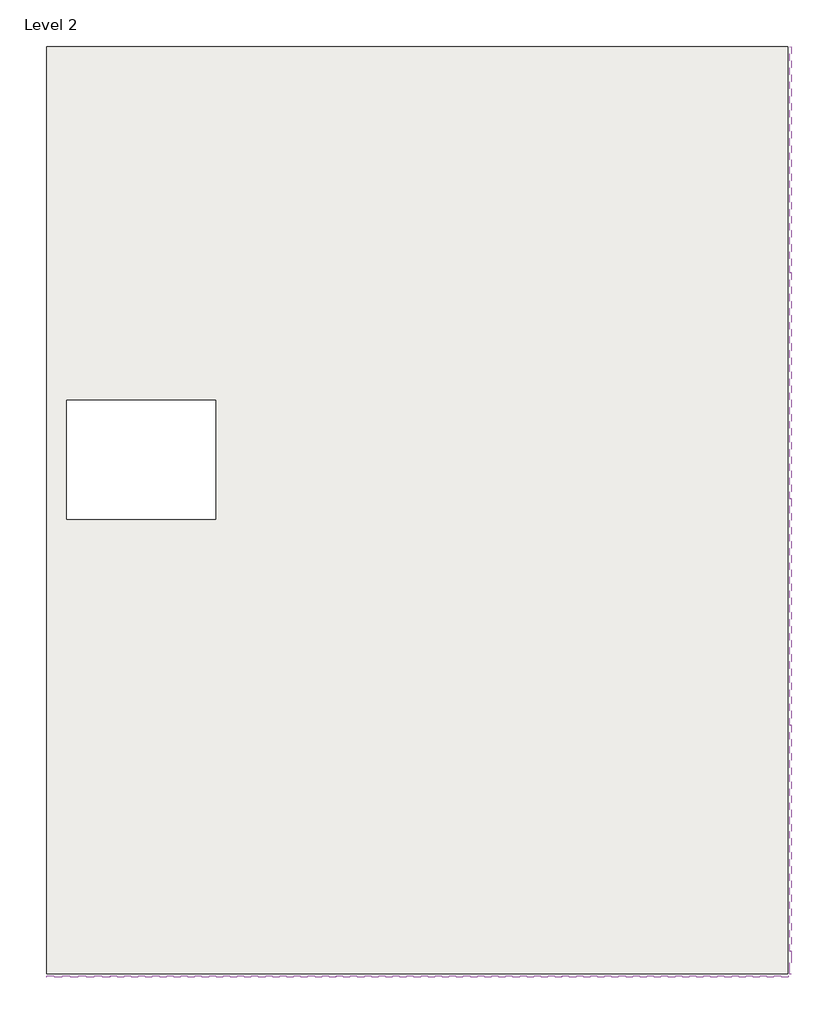
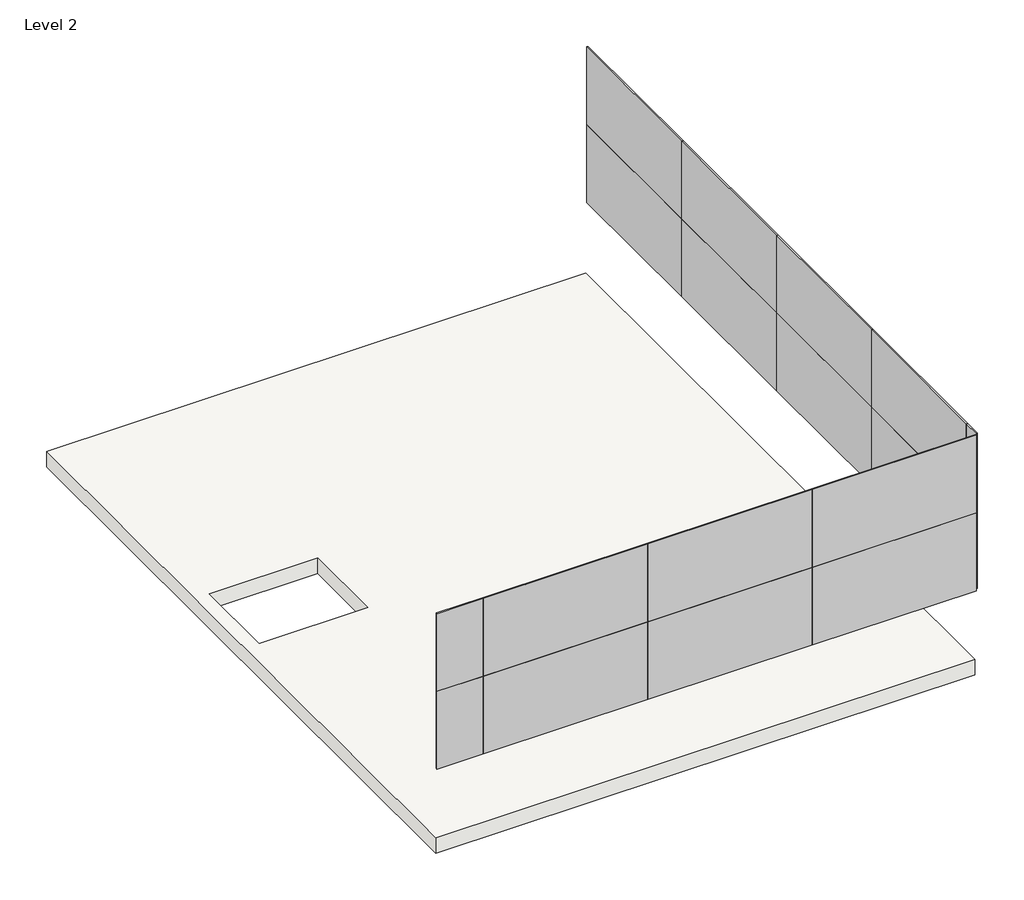
# One storey: 18 plates, 1 slab.
"""IFC4 building model written with IfcOpenShell, lengths in millimetres."""

import ifcopenshell
import ifcopenshell.guid

model = None  # the IFC model being written
_history = None  # IfcOwnerHistory: only IFC2X3 demands one
_inside = {}  # id of a spatial element -> (the spatial element, [elements in it])
_under = {}  # id of a project, library or spatial element -> (it, [spatial elements below it])
_declared = {}  # id of a project -> (the project, [libraries it declares])
_typed = {}  # id of a type object -> (the type object, [elements of that type])
_made_of = {}  # id of a material, layer set ... -> (it, [elements and type objects made of it])


def new_model(schema):
    """Start an empty IFC model of exactly this schema.

    Asked for "IFC4X3", IfcOpenShell would pick the latest addendum, in which some entities
    have other attributes; the version numbers below select the first issue.
    IFC2X3 requires an IfcOwnerHistory on every rooted entity: one is made here for all.
    """
    global model, _history
    if schema == "IFC4X3":
        model = ifcopenshell.file(schema_version=(4, 3, 0, 0))
    else:
        model = ifcopenshell.file(schema=schema)
    _inside.clear()
    _under.clear()
    _declared.clear()
    _typed.clear()
    _made_of.clear()
    _history = None
    if model.schema == "IFC2X3":
        org = make("IfcOrganization", Name="unknown")
        user = make(
            "IfcPersonAndOrganization",
            ThePerson=make("IfcPerson", FamilyName="unknown"),
            TheOrganization=org,
        )
        app = make(
            "IfcApplication",
            ApplicationDeveloper=org,
            Version="unknown",
            ApplicationFullName="unknown",
            ApplicationIdentifier="unknown",
        )
        _history = make(
            "IfcOwnerHistory",
            OwningUser=user,
            OwningApplication=app,
            ChangeAction="ADDED",
            CreationDate=0,
        )
    return model


def make(cls, **values):
    """One entity of the class cls with the attributes given. An attribute that is None is left unset."""
    return model.create_entity(
        cls, **{name: value for name, value in values.items() if value is not None}
    )


def rooted(cls, **values):
    """An entity with a GlobalId (a new one), such as an element, a storey or a relation."""
    return make(cls, GlobalId=ifcopenshell.guid.new(), OwnerHistory=_history, **values)


def si_unit(unit_type, name, prefix=None):
    """IfcSIUnit, for example si_unit("LENGTHUNIT", "METRE", prefix="MILLI")."""
    return make("IfcSIUnit", UnitType=unit_type, Prefix=prefix, Name=name)


def assignment(units):
    """IfcUnitAssignment: the units of a project."""
    return None if units is None else make("IfcUnitAssignment", Units=units)


def point(xyz):
    """IfcCartesianPoint."""
    return None if xyz is None else make("IfcCartesianPoint", Coordinates=xyz)


def direction(xyz):
    """IfcDirection."""
    return None if xyz is None else make("IfcDirection", DirectionRatios=xyz)


def frame(location, z_axis=None, x_axis=None):
    """IfcAxis2Placement3D, a coordinate frame: its origin and axes. An axis left out is left unset."""
    return make(
        "IfcAxis2Placement3D",
        Location=point(location),
        Axis=direction(z_axis),
        RefDirection=direction(x_axis),
    )


def origin():
    """The frame at (0, 0, 0) with its axes left unset."""
    return frame((0.0, 0.0, 0.0))


def origin_with_axes():
    """The frame at (0, 0, 0) with the z axis (0, 0, 1) and the x axis (1, 0, 0) written out."""
    return frame((0.0, 0.0, 0.0), z_axis=(0.0, 0.0, 1.0), x_axis=(1.0, 0.0, 0.0))


def place(relative_to, where):
    """IfcLocalPlacement: puts the frame where relative to a parent placement (None: the world)."""
    return make(
        "IfcLocalPlacement", PlacementRelTo=relative_to, RelativePlacement=where
    )


def context(
    kind, dimensions, precision=None, world=None, true_north=None, identifier=None
):
    """IfcGeometricRepresentationContext, for example the 3D "Model" context."""
    return make(
        "IfcGeometricRepresentationContext",
        ContextIdentifier=identifier,
        ContextType=kind,
        CoordinateSpaceDimension=dimensions,
        Precision=precision,
        WorldCoordinateSystem=world,
        TrueNorth=true_north,
    )


def project(units=None, contexts=None):
    """IfcProject with its units and contexts."""
    return rooted(
        "IfcProject",
        Name="project",
        RepresentationContexts=contexts,
        UnitsInContext=assignment(units),
    )


def spatial(cls, under=None, at=None, **own):
    """A site, building, storey or space (cls), placed at a placement, below another one or the project."""
    s = rooted(cls, ObjectPlacement=at, **own)
    if under is not None:
        _under.setdefault(under.id(), (under, []))[1].append(s)
    return s


def polyline(points):
    """IfcPolyline through the points."""
    return make("IfcPolyline", Points=[point(p) for p in points])


def outline(outer, holes=None, kind="AREA"):
    """IfcArbitraryClosedProfileDef: a profile drawn as a closed curve; with holes, ...WithVoids."""
    if holes is None:
        return make("IfcArbitraryClosedProfileDef", ProfileType=kind, OuterCurve=outer)
    return make(
        "IfcArbitraryProfileDefWithVoids",
        ProfileType=kind,
        OuterCurve=outer,
        InnerCurves=holes,
    )


def extrude(swept, where, along, depth):
    """IfcExtrudedAreaSolid: the profile swept, set in the frame where, extruded along a direction by depth."""
    return make(
        "IfcExtrudedAreaSolid",
        SweptArea=swept,
        Position=where,
        ExtrudedDirection=direction(along),
        Depth=depth,
    )


def shape(context_of_items, identifier, shape_type, items):
    """IfcShapeRepresentation: the items that make up one representation, for example the "Body"."""
    return make(
        "IfcShapeRepresentation",
        ContextOfItems=context_of_items,
        RepresentationIdentifier=identifier,
        RepresentationType=shape_type,
        Items=items,
    )


def source(mapping_origin, context_of_items, identifier, shape_type, items):
    """IfcRepresentationMap: a shape defined once, which mapped items show again and again."""
    return make(
        "IfcRepresentationMap",
        MappingOrigin=mapping_origin,
        MappedRepresentation=shape(context_of_items, identifier, shape_type, items),
    )


def transform(
    local_origin,
    x_axis=None,
    y_axis=None,
    z_axis=None,
    scale=None,
    scale2=None,
    scale3=None,
    uniform=True,
):
    """IfcCartesianTransformationOperator3D, or its non-uniform kind. x_axis, y_axis, z_axis: its Axis1, 2, 3."""
    if uniform:
        return make(
            "IfcCartesianTransformationOperator3D",
            Axis1=direction(x_axis),
            Axis2=direction(y_axis),
            LocalOrigin=point(local_origin),
            Scale=scale,
            Axis3=direction(z_axis),
        )
    return make(
        "IfcCartesianTransformationOperator3DnonUniform",
        Axis1=direction(x_axis),
        Axis2=direction(y_axis),
        LocalOrigin=point(local_origin),
        Scale=scale,
        Axis3=direction(z_axis),
        Scale2=scale2,
        Scale3=scale3,
    )


def mapped(mapping_source, mapping_target):
    """IfcMappedItem: shows the shape of a source again, moved by a transform."""
    return make(
        "IfcMappedItem", MappingSource=mapping_source, MappingTarget=mapping_target
    )


def made_of(thing, what):
    """Note that an element or type object is made of a material, layer set ...; save() writes the relation."""
    if what is not None:
        _made_of.setdefault(what.id(), (what, []))[1].append(thing)
    return thing


def element(
    cls,
    number,
    at=None,
    inside=None,
    cuts=None,
    type_object=None,
    material=None,
    context=None,
    identifier="Body",
    shape_type=None,
    held_by="IfcProductDefinitionShape",
    body=None,
    shapes=None,
    **own,
):
    """One element of the class cls, such as IfcWall. Its Tag is "e" and its number.

    at: its placement. inside: the storey or other place that contains it. cuts: it is an
    opening in that element (IfcRelVoidsElement). A single representation is given by context,
    identifier, shape_type and body (its items); several are given by shapes. held_by: the class
    of the entity that holds the representations. save() writes the other relations.
    """
    e = rooted(cls, Tag="e%d" % number, ObjectPlacement=at, **own)
    if body is not None:
        shapes = [shape(context, identifier, shape_type, body)]
    if shapes is not None:
        e.Representation = make(held_by, Representations=shapes)
    if inside is not None:
        _inside.setdefault(inside.id(), (inside, []))[1].append(e)
    if cuts is not None:
        rooted(
            "IfcRelVoidsElement", RelatingBuildingElement=cuts, RelatedOpeningElement=e
        )
    if type_object is not None:
        _typed.setdefault(type_object.id(), (type_object, []))[1].append(e)
    return made_of(e, material)


def aggregate(whole, parts):
    """IfcRelAggregates: a whole, such as a stair, and the parts it consists of."""
    return rooted("IfcRelAggregates", RelatingObject=whole, RelatedObjects=parts)


def save(model, path):
    """Write the relations noted so far, then the file.

    IfcRelAggregates (storeys below a building ...), IfcRelContainedInSpatialStructure (elements
    in a storey), IfcRelDefinesByType, IfcRelAssociatesMaterial and IfcRelDeclares: one each for
    every whole, place, type object, material and project.
    """
    for whole, parts in _under.values():
        aggregate(whole, parts)
    for where, things in _inside.values():
        rooted(
            "IfcRelContainedInSpatialStructure",
            RelatedElements=things,
            RelatingStructure=where,
        )
    for kind, things in _typed.values():
        rooted("IfcRelDefinesByType", RelatedObjects=things, RelatingType=kind)
    for what, things in _made_of.values():
        rooted("IfcRelAssociatesMaterial", RelatedObjects=things, RelatingMaterial=what)
    for by, libraries in _declared.values():
        rooted("IfcRelDeclares", RelatingContext=by, RelatedDefinitions=libraries)
    model.write(path)


def system_panel_glazed_1e57f9bb(model_context):
    return source(origin(), model_context, "Body", "SweptSolid", [
        extrude(outline(polyline([(1524.0000002, 19.05), (-1524.0000002, 19.05), (-1524.0000002, 44.45), (1524.0000002, 44.45), (1524.0000002, 19.05)])), origin_with_axes(), (0.0, 0.0, 1.0), 1524.0),
    ])


def system_panel_glazed_ccfd9adb(model_context):
    return source(origin(), model_context, "Body", "SweptSolid", [
        extrude(outline(polyline([(427.9999998, 19.05), (-427.9999998, 19.05), (-427.9999998, 44.45), (427.9999998, 44.45), (427.9999998, 19.05)])), origin_with_axes(), (0.0, 0.0, 1.0), 1524.0),
    ])


def system_panel_glazed_88f24eba(model_context):
    return source(origin(), model_context, "Body", "SweptSolid", [
        extrude(outline(polyline([(153.9999998, 19.05), (-153.9999998, 19.05), (-153.9999998, 44.45), (153.9999998, 44.45), (153.9999998, 19.05)])), origin_with_axes(), (0.0, 0.0, 1.0), 1524.0),
    ])


model = new_model("IFC4")

# Units and contexts
model_context = context("Model", 3, world=origin())
ifc_project = project(units=[si_unit("LENGTHUNIT", "METRE", prefix="MILLI")], contexts=[model_context])

# Site, building, storey
site = spatial("IfcSite", under=ifc_project)
building = spatial("IfcBuilding", under=site)
storey = spatial("IfcBuildingStorey", under=building, Name="Level 2", Elevation=3200.0)

# Plates
placement = place(None, origin())
system_panel_glazed_shape = system_panel_glazed_1e57f9bb(model_context)
element("IfcPlate", 1, ObjectType="System Panel : Glazed", at=placement, inside=storey, context=model_context, shape_type="MappedRepresentation", body=[
    mapped(system_panel_glazed_shape, transform((2137.6340362, 1399.6955828, 4572.0), x_axis=(-1.0, 0.0, 0.0), y_axis=(0.0, -1.0, 0.0), z_axis=(0.0, 0.0, 1.0))),
])
element("IfcPlate", 2, ObjectType="System Panel : Glazed", at=placement, inside=storey, context=model_context, shape_type="MappedRepresentation", body=[
    mapped(system_panel_glazed_shape, transform((-910.3659639, 1399.6955828, 4572.0), x_axis=(-1.0, 0.0, 0.0), y_axis=(0.0, -1.0, 0.0), z_axis=(0.0, 0.0, 1.0))),
])
element("IfcPlate", 3, ObjectType="System Panel : Glazed", at=placement, inside=storey, context=model_context, shape_type="MappedRepresentation", body=[
    mapped(system_panel_glazed_shape, transform((-3958.3659639, 1399.6955828, 4572.0), x_axis=(-1.0, 0.0, 0.0), y_axis=(0.0, -1.0, 0.0), z_axis=(0.0, 0.0, 1.0))),
])
element("IfcPlate", 4, ObjectType="System Panel : Glazed", at=placement, inside=storey, context=model_context, shape_type="MappedRepresentation", body=[
    mapped(system_panel_glazed_shape, transform((2137.6340362, 1399.6955828, 6096.0), x_axis=(-1.0, 0.0, 0.0), y_axis=(0.0, -1.0, 0.0), z_axis=(0.0, 0.0, 1.0))),
])
element("IfcPlate", 5, ObjectType="System Panel : Glazed", at=placement, inside=storey, context=model_context, shape_type="MappedRepresentation", body=[
    mapped(system_panel_glazed_shape, transform((-910.3659639, 1399.6955828, 6096.0), x_axis=(-1.0, 0.0, 0.0), y_axis=(0.0, -1.0, 0.0), z_axis=(0.0, 0.0, 1.0))),
])
element("IfcPlate", 6, ObjectType="System Panel : Glazed", at=placement, inside=storey, context=model_context, shape_type="MappedRepresentation", body=[
    mapped(system_panel_glazed_shape, transform((-3958.3659639, 1399.6955828, 6096.0), x_axis=(-1.0, 0.0, 0.0), y_axis=(0.0, -1.0, 0.0), z_axis=(0.0, 0.0, 1.0))),
])
element("IfcPlate", 7, ObjectType="System Panel : Glazed", at=placement, inside=storey, context=model_context, shape_type="MappedRepresentation", body=[
    mapped(system_panel_glazed_shape, transform((3661.6340364, 12375.6955827, 4572.0), x_axis=(0.0, -1.0, 0.0), y_axis=(1.0, 0.0, 0.0), z_axis=(0.0, 0.0, 1.0))),
])
element("IfcPlate", 8, ObjectType="System Panel : Glazed", at=placement, inside=storey, context=model_context, shape_type="MappedRepresentation", body=[
    mapped(system_panel_glazed_shape, transform((3661.6340364, 9327.6955825, 4572.0), x_axis=(0.0, -1.0, 0.0), y_axis=(1.0, 0.0, 0.0), z_axis=(0.0, 0.0, 1.0))),
])
element("IfcPlate", 9, ObjectType="System Panel : Glazed", at=placement, inside=storey, context=model_context, shape_type="MappedRepresentation", body=[
    mapped(system_panel_glazed_shape, transform((3661.6340364, 6279.6955825, 4572.0), x_axis=(0.0, -1.0, 0.0), y_axis=(1.0, 0.0, 0.0), z_axis=(0.0, 0.0, 1.0))),
])
element("IfcPlate", 10, ObjectType="System Panel : Glazed", at=placement, inside=storey, context=model_context, shape_type="MappedRepresentation", body=[
    mapped(system_panel_glazed_shape, transform((3661.6340364, 3231.6955825, 4572.0), x_axis=(0.0, -1.0, 0.0), y_axis=(1.0, 0.0, 0.0), z_axis=(0.0, 0.0, 1.0))),
])
element("IfcPlate", 11, ObjectType="System Panel : Glazed", at=placement, inside=storey, context=model_context, shape_type="MappedRepresentation", body=[
    mapped(system_panel_glazed_shape, transform((3661.6340364, 12375.6955827, 6096.0), x_axis=(0.0, -1.0, 0.0), y_axis=(1.0, 0.0, 0.0), z_axis=(0.0, 0.0, 1.0))),
])
element("IfcPlate", 12, ObjectType="System Panel : Glazed", at=placement, inside=storey, context=model_context, shape_type="MappedRepresentation", body=[
    mapped(system_panel_glazed_shape, transform((3661.6340364, 9327.6955825, 6096.0), x_axis=(0.0, -1.0, 0.0), y_axis=(1.0, 0.0, 0.0), z_axis=(0.0, 0.0, 1.0))),
])
element("IfcPlate", 13, ObjectType="System Panel : Glazed", at=placement, inside=storey, context=model_context, shape_type="MappedRepresentation", body=[
    mapped(system_panel_glazed_shape, transform((3661.6340364, 6279.6955825, 6096.0), x_axis=(0.0, -1.0, 0.0), y_axis=(1.0, 0.0, 0.0), z_axis=(0.0, 0.0, 1.0))),
])
element("IfcPlate", 14, ObjectType="System Panel : Glazed", at=placement, inside=storey, context=model_context, shape_type="MappedRepresentation", body=[
    mapped(system_panel_glazed_shape, transform((3661.6340364, 3231.6955825, 6096.0), x_axis=(0.0, -1.0, 0.0), y_axis=(1.0, 0.0, 0.0), z_axis=(0.0, 0.0, 1.0))),
])
system_panel_glazed_2_shape = system_panel_glazed_ccfd9adb(model_context)
element("IfcPlate", 15, ObjectType="System Panel : Glazed", at=placement, inside=storey, context=model_context, shape_type="MappedRepresentation", body=[
    mapped(system_panel_glazed_2_shape, transform((-5910.3659638, 1399.6955828, 4572.0), x_axis=(-1.0, 0.0, 0.0), y_axis=(0.0, -1.0, 0.0), z_axis=(0.0, 0.0, 1.0))),
])
element("IfcPlate", 16, ObjectType="System Panel : Glazed", at=placement, inside=storey, context=model_context, shape_type="MappedRepresentation", body=[
    mapped(system_panel_glazed_2_shape, transform((-5910.3659638, 1399.6955828, 6096.0), x_axis=(-1.0, 0.0, 0.0), y_axis=(0.0, -1.0, 0.0), z_axis=(0.0, 0.0, 1.0))),
])
system_panel_glazed_3_shape = system_panel_glazed_88f24eba(model_context)
element("IfcPlate", 17, ObjectType="System Panel : Glazed", at=placement, inside=storey, context=model_context, shape_type="MappedRepresentation", body=[
    mapped(system_panel_glazed_3_shape, transform((3661.6340364, 1553.6955827, 4572.0), x_axis=(0.0, -1.0, 0.0), y_axis=(1.0, 0.0, 0.0), z_axis=(0.0, 0.0, 1.0))),
])
element("IfcPlate", 18, ObjectType="System Panel : Glazed", at=placement, inside=storey, context=model_context, shape_type="MappedRepresentation", body=[
    mapped(system_panel_glazed_3_shape, transform((3661.6340364, 1553.6955827, 6096.0), x_axis=(0.0, -1.0, 0.0), y_axis=(1.0, 0.0, 0.0), z_axis=(0.0, 0.0, 1.0))),
])

# Slab
element("IfcSlab", 19, ObjectType="Generic - 12\"", at=placement, inside=storey, context=model_context, shape_type="SweptSolid", body=[
    extrude(outline(polyline([(-6335.3659636, 1402.6955828), (-6335.3659636, 13896.6955828), (3658.6340364, 13896.6955828), (3658.6340364, 1402.6955828), (-6335.3659636, 1402.6955828)]), holes=[polyline([(-4059.8993101, 7527.9023719), (-4059.8993101, 9133.9023719), (-6065.8993101, 9133.9023719), (-6065.8993101, 7527.9023719), (-4059.8993101, 7527.9023719)])]), frame((0.0, 0.0, 2895.2), z_axis=(0.0, 0.0, 1.0), x_axis=(1.0, 0.0, 0.0)), (0.0, 0.0, 1.0), 304.8),
])

save(model, "model.ifc")

# Revit data of these elements
# Type "System Panel : Glazed"
#   Construction Type Id = "GSP4R"
#   Analytic Construction = "1/8 in Pilkington single glazing"
#   Visual Light Transmittance = 0.9
#   Solar Heat Gain Coefficient = 0.86
#   Heat Transfer Coefficient (U) = 6.7069 W/(m²·K)
# Type "Generic - 12\""
#   Assembly Code = "B1010"
#   Function = 0
#   Layers, outside or top first: 0.3048 m no material (function 1)
# Elements 1, 2, 3, 4, 5, 6, 7, 8, 9, 10, 11, 12, 13, 14, 15, 16, 17, 18 (IfcPlate, "System Panel : Glazed")
#   Phase Created = New Construction
#   Materials on its faces: "Glass"
# Element 19 (IfcSlab, "Generic - 12\"")
#   built-in parameter 1001955 = -1.5708 (stored number, unit not read)
#   Height Offset From Level = 0.00 m
#   Phase Created = New Construction
#   Materials on its faces: "Default Floor"
# Materials
#   "Glass": class "Glass", colour RGB 0 128 192, transparency 0.75, Description = "Soda Lime Glass", Cost = 0
#   "Default Floor": class "Miscellaneous", colour RGB 128 128 128, transparency 0, Cost = 0
